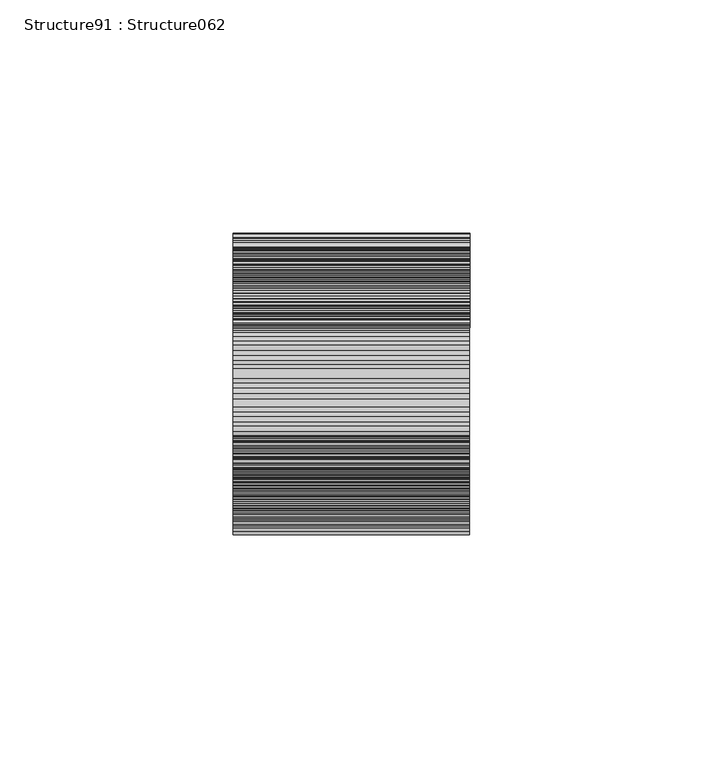
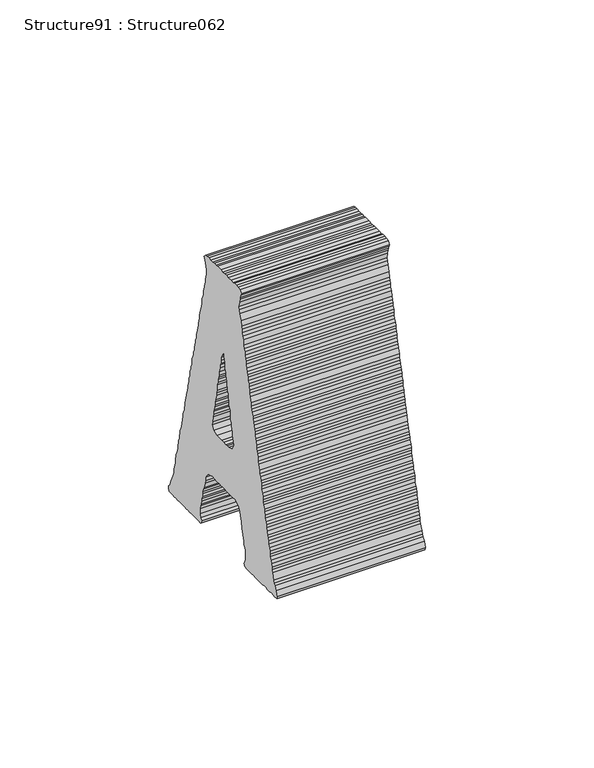
"""IFC4 building model written with IfcOpenShell, lengths in millimetres: proxy geometry, Structure91 : Structure062."""

from ifc_helpers import new_model, si_unit, frame, origin, place, context, project, spatial, polyline, outline, extrude, source, transform, mapped, element, save


def structure91_structure062_a9b4e26e(model_context):
    return source(origin(), model_context, "Body", "SweptSolid", [
        extrude(outline(polyline([(0.9094651, 0.0), (2.0811665, -0.5191353), (2.9906316, -0.6475848), (4.1562841, -0.7760343), (5.1991801, -1.1663641), (5.9748585, -1.299795), (7.1504738, -1.6851436), (8.1894559, -1.6851436), (9.3551083, -2.0758292), (10.2645735, -2.3377097), (11.4362748, -2.5946087), (12.3453841, -2.8564891), (13.3818755, -2.9849385), (14.1582655, -3.3752685), (15.4626861, -3.5040738), (16.3721513, -3.5040738), (17.5385154, -3.7659542), (19.491944, -4.4181645), (20.2718921, -4.6750635), (21.3101626, -4.9369439), (22.3470097, -4.9369439), (23.2561191, -5.1941988), (24.4278204, -5.5845286), (25.4700048, -5.9748585), (26.6363689, -5.9748585), (27.4124031, -6.3651884), (28.7175354, -6.6220874), (30.535754, -7.0127732), (31.5743802, -7.1462041), (32.7400327, -7.403103), (33.6555467, -7.7934329), (35.4741211, -7.7934329), (36.5102567, -7.5315525), (37.5492387, -7.2746536), (38.3288311, -6.8843236), (39.3671015, -6.3651884), (40.4099976, -7.2746536), (40.5395145, -8.1837629), (40.5395145, -9.093228), (40.2826155, -10.2645735), (40.2826155, -11.3021323), (40.5395145, -12.4684964), (40.4099976, -13.2491562), (40.5395145, -14.1586213), (40.5395145, -16.2390762), (40.2826155, -17.2769908), (40.2826155, -18.319531), (40.5395145, -19.4858951), (40.4099976, -20.6572406), (40.4099976, -22.3423842), (40.2826155, -23.5137297), (40.5395145, -24.422839), (40.5395145, -25.5941846), (40.4099976, -26.5032939), (40.2826155, -27.6746394), (39.2382962, -28.4506736), (38.3288311, -27.9315383), (37.4197218, -27.6746394), (36.6397736, -27.5412085), (35.4741211, -27.2843095), (33.5199809, -26.8939796), (32.6112274, -27.1508785), (31.4448633, -27.412759), (29.3636968, -28.1934188), (27.545834, -28.4506736), (26.5089869, -28.712554), (25.3372855, -28.8410035), (24.2943895, -29.102884), (23.2561191, -29.6216633), (21.3101626, -29.7501128), (20.2718921, -30.012349), (19.491944, -30.5311284), (18.3202426, -30.5311284), (17.2816164, -30.9214583), (16.3721513, -31.1833388), (15.3356599, -31.1833388), (14.1582655, -31.4402377), (13.1253323, -31.8309234), (12.2158672, -32.2212534), (11.4362748, -32.3497029), (10.2645735, -32.4781523), (9.3551083, -32.8684823), (8.1894559, -32.8684823), (7.1504738, -33.259168), (6.2374505, -33.3876175), (5.0714422, -33.6494978), (3.2475306, -34.2967268), (2.0811665, -34.2967268), (1.1720572, -34.5586071), (0.1334309, -34.815862), (-1.0382704, -35.3396228), (-1.8178628, -35.4680723), (-2.8568449, -35.7249713), (-3.8990293, -35.8584022), (-5.0653934, -36.2487321), (-5.8471206, -36.505987), (-7.0166871, -36.505987), (-8.1826954, -36.8963168), (-8.9644226, -37.0297477), (-10.1364798, -37.4150963), (-11.1690572, -37.5485272), (-12.2115974, -37.6769767), (-12.9915456, -37.938857), (-14.03373, -38.3245613), (-15.3292552, -38.4579923), (-16.3678815, -38.7148913), (-18.1861001, -39.1052211), (-19.3581573, -39.3671016), (-20.2672666, -39.7528059), (-21.4371888, -40.0146862), (-22.2189161, -40.2765667), (-23.1223323, -40.5334657), (-24.1648726, -40.5334657), (-25.465735, -41.0572265), (-26.5025822, -41.3141255), (-27.4173846, -41.4429308), (-28.4560108, -41.4429308), (-29.235959, -41.7048112), (-30.5311284, -42.0951412), (-31.3110766, -42.2235906), (-32.3536168, -42.6139205), (-33.5214042, -42.6139205), (-34.4308693, -43.1330558), (-35.3399786, -43.3949361), (-36.37647, -43.3949361), (-37.5424783, -43.6568165), (-38.7202285, -44.0421651), (-39.6236447, -44.3040455), (-40.405372, -44.5659258), (-41.5752942, -44.6897497), (-42.6139205, -45.0850611), (-43.7856218, -45.3419601), (-44.8221132, -45.3419601), (-45.7372714, -45.4704095), (-46.6406876, -45.9941704), (-47.812389, -46.2510694), (-48.8510152, -46.5133056), (-49.7601245, -46.5133056), (-50.6731478, -46.9036355), (-52.8777823, -47.5508643), (-53.7929405, -47.9411943), (-54.5689747, -48.33188), (-55.738897, -49.1125398), (-57.5532016, -49.7601246), (-58.4665807, -49.5028698), (-58.5957419, -48.1984491), (-58.4665807, -47.4224149), (-58.3331498, -46.2510694), (-58.5957419, -45.2135106), (-58.5957419, -44.0421651), (-58.3331498, -43.0042505), (-58.3331498, -42.0951412), (-58.4665807, -41.0572265), (-58.4665807, -40.1481171), (-58.5957419, -38.8433407), (-58.5957419, -37.938857), (-58.4665807, -36.8963168), (-58.3331498, -35.7249713), (-58.5957419, -34.815862), (-58.5957419, -31.8309234), (-58.3331498, -30.6595779), (-57.4297336, -30.1407986), (-56.6480063, -30.5311284), (-55.6115149, -30.7880274), (-53.3972734, -30.7880274), (-52.3586471, -30.7880274), (-51.4495378, -30.5311284), (-50.6731478, -30.1407986), (-49.3683714, -30.012349), (-48.4592621, -29.7501128), (-47.5497969, -29.3597829), (-46.6406876, -29.102884), (-45.6038405, -28.8410035), (-43.2661308, -28.5841045), (-41.5752942, -27.9315383), (-40.2762109, -27.6746394), (-38.9767716, -27.022429), (-38.1950444, -26.1129639), (-37.4190102, -24.6847195), (-37.6759092, -23.6471607), (-37.6759092, -21.5663499), (-37.5424783, -20.2669108), (-37.5424783, -17.5388712), (-37.6759092, -16.3675257), (-37.4190102, -15.4584164), (-37.5424783, -14.4205018), (-37.6759092, -13.3825871), (-37.5424783, -12.4684964), (-37.4190102, -11.1736828), (-37.6759092, -10.393023), (-38.0676623, -8.836329), (-38.8476105, -8.050332), (-40.2762109, -7.0127732), (-41.4422191, -7.0127732), (-42.6139205, -6.7555183), (-44.561656, -6.236739), (-45.3472973, -5.7129781), (-46.5133056, -5.4560791), (-47.2932538, -5.3276297), (-48.33188, -5.3276297), (-49.3683714, -4.803513), (-50.4126907, -4.6750635), (-51.4495378, -4.546614), (-52.3586471, -4.156284), (-53.6595096, -3.7659542), (-55.3489229, -3.8944037), (-56.6480063, -4.2847336), (-57.2966585, -4.9369439), (-58.5957419, -4.156284), (-58.4665807, -2.9849385), (-58.3331498, -1.9473798), (-58.3331498, 0.1334309), (-58.4665807, 1.1709897), (-58.4665807, 2.2089043), (-58.3331498, 3.1183694), (-58.4665807, 4.0274787), (-58.4665807, 5.3272738), (-58.3331498, 6.1079336), (-58.4665807, 7.4077286), (-58.3331498, 8.1887442), (-58.5957419, 9.226303), (-58.3331498, 10.3976485), (-58.5957419, 11.5640127), (-58.4665807, 12.473122), (-58.3331498, 13.516018), (-58.3331498, 14.5535768), (-57.2966585, 14.9442625), (-56.3875492, 14.6823821), (-55.738897, 14.0347974), (-54.5689747, 13.772917), (-53.7929405, 13.382587), (-52.6151903, 12.8634519), (-50.6731478, 11.9543426), (-49.8875066, 11.6974436), (-48.5941162, 11.5640127), (-47.5497969, 11.3067578), (-46.6406876, 11.0448775), (-45.8646534, 10.6545476), (-44.5616561, 10.526098), (-42.6139205, 10.2642176), (-41.4422191, 9.8788692), (-40.5384471, 9.483202), (-39.6236447, 9.226303), (-38.4576364, 9.0978535), (-37.4190102, 8.9644226), (-36.5059869, 8.8359732), (-35.6004358, 8.3171937), (-34.2956593, 8.1887442), (-33.3922431, 8.0553133), (-32.3536168, 7.926508), (-31.4405935, 7.5361781), (-30.4019673, 7.1458482), (-29.235959, 6.8889491), (-27.5447666, 6.6270688), (-26.3752002, 6.2363831), (-25.203143, 6.1079336), (-24.4235506, 5.8510345), (-23.3849244, 5.4557233), (-22.4793732, 5.3272738), (-21.3037579, 4.9419252), (-20.2672666, 4.9419252), (-19.3581573, 4.679689), (-18.319531, 4.4227901), (-17.1474738, 4.1609097), (-15.2018732, 3.6371488), (-14.1632469, 3.3802499), (-13.1207067, 3.3802499), (-12.2115974, 2.9895641), (-11.3024881, 2.5992342), (-10.0012698, 2.5992342), (-9.2270147, 2.0804548), (-8.1826954, 2.0804548), (-7.0166871, 1.9520053), (-5.9745027, 1.4328701), (-5.0653934, 1.4328701), (-4.1619771, 0.9140907), (-2.8568449, 0.7806598), (-1.9473797, 0.7806598), (-0.7817273, 0.2618804), (0.0, 0.0), (0.9094651, 0.0)]), holes=[polyline([(-20.9137838, -13.9017224), (-20.9137838, -16.8866609), (-20.7903157, -18.0576507), (-21.0472147, -19.2289962), (-20.7903157, -20.1384613), (-20.9137838, -21.0475706), (-20.2672666, -22.9945945), (-18.5817672, -23.6471607), (-17.2809048, -23.3852802), (-16.3678815, -23.123044), (-15.4623303, -22.866145), (-14.1632469, -22.9945945), (-13.2480888, -22.4758151), (-12.2115974, -22.3423842), (-11.3024881, -22.2139347), (-10.393023, -21.8285862), (-9.3508386, -21.6951552), (-8.3122123, -21.6951552), (-7.146204, -21.5663499), (-6.3644768, -21.1760201), (-5.3276296, -20.9141397), (-4.2854452, -20.9141397), (-3.117302, -20.3953602), (-1.9473797, -20.3953602), (-1.0382704, -20.0050304), (-0.2561874, -19.8762251), (1.0389821, -19.7477755), (2.0811665, -19.4858951), (3.1180136, -19.2289962), (4.0274787, -19.0955653), (5.0714422, -19.0955653), (6.1082894, -18.5767858), (7.0177545, -18.4483363), (8.1894559, -18.4483363), (9.2216774, -18.0576507), (10.1368356, -17.8007516), (11.0463007, -17.8007516), (10.1368356, -17.1485414), (9.0928721, -16.7582114), (8.056025, -16.6294061), (6.8900167, -16.6294061), (6.1082894, -16.1106266), (4.9365881, -15.9771957), (3.1180136, -15.4584164), (1.8189302, -15.3299669), (0.9094651, -15.2015173), (0.0, -14.9392811), (-1.0382704, -14.8108317), (-2.2078369, -14.4205018), (-4.2854452, -14.2920522), (-5.3276296, -14.0301718), (-6.3644768, -13.9017224), (-8.1826954, -13.5113925), (-9.2270147, -12.9922572), (-10.2638619, -12.9922572), (-11.1690572, -12.7303769), (-12.3446725, -12.6019274), (-13.1207067, -12.2115974), (-14.286715, -12.2115974), (-15.4623303, -11.8212675), (-17.2809048, -11.5590313), (-18.5817672, -11.3021323), (-20.1377496, -12.0831479), (-20.9137838, -13.9017224)])]), frame((-56111.3901178, 291548.157521, -317.0048136), z_axis=(-0.9999998917542984, 0.00046528635450596156, 0.0), x_axis=(0.0, 0.0, 1.0)), (0.0, 0.0, 1.0), 50.8),
    ])


if __name__ == "__main__":
    model = new_model("IFC4")
    model_context = context("Model", 3, world=origin())
    ifc_project = project(units=[si_unit("LENGTHUNIT", "METRE", prefix="MILLI")], contexts=[model_context])
    site = spatial("IfcSite", under=ifc_project)
    building = spatial("IfcBuilding", under=site)
    placement = place(None, origin())
    structure91_structure062_shape = structure91_structure062_a9b4e26e(model_context)
    element("IfcBuildingElementProxy", 1, Name="Structure91 : Structure062", ObjectType="Structure91 : Structure062", at=placement, inside=building, context=model_context, shape_type="MappedRepresentation", body=[
        mapped(structure91_structure062_shape, transform((0.0, 0.0, 0.0), x_axis=(1.0, 0.0, 0.0), y_axis=(0.0, 1.0, 0.0), z_axis=(0.0, 0.0, 1.0))),
    ])
    save(model, "model.ifc")

# Revit data of these elements
# Type "Structure91 : Structure062"
#   NameOverride = "Structure062"
# Element 1 (IfcBuildingElementProxy, "Structure91 : Structure062")
#   Materials on its faces: "BRUSHED ALUMINUM LETTERING"
# Materials
#   "BRUSHED ALUMINUM LETTERING": class "Unassigned", colour RGB 169 181 186, transparency 0, Cost = 0
